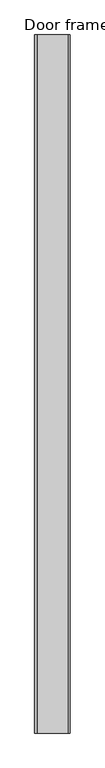
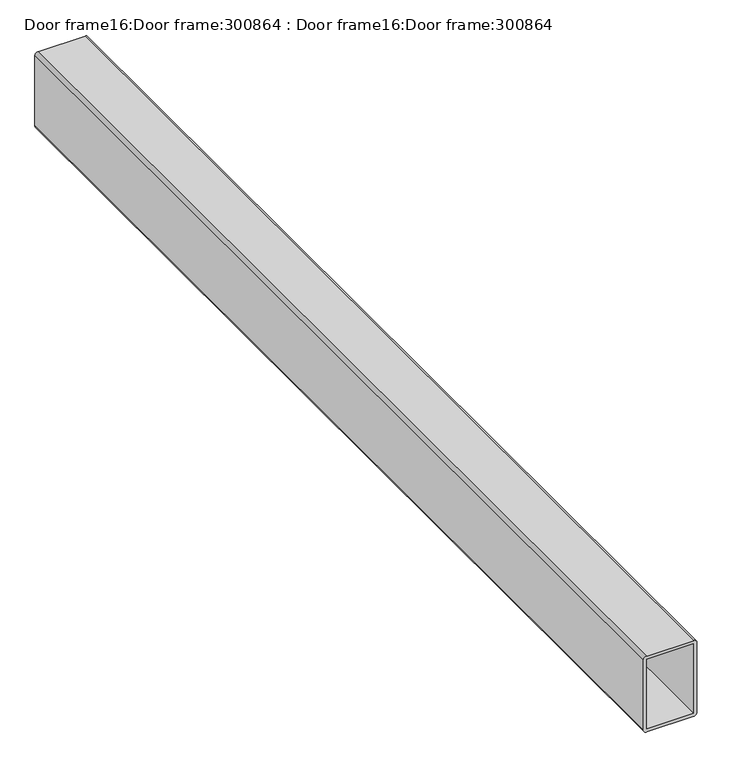
"""IFC4 building model written with IfcOpenShell, lengths in millimetres: proxy geometry, Door frame16:Door frame:300864 : Door frame16:Door frame:300864."""

from ifc_helpers import new_model, si_unit, point, frame, frame_2d, origin, place, context, project, spatial, polyline, circle_curve, trimmed, segment, composite_curve, outline, extrude, source, transform, mapped, element, save


def door_frame16_door_frame_300864_door_frame16_door_frame_4405bbaf(model_context):
    return source(origin(), model_context, "Body", "SweptSolid", [
        extrude(outline(composite_curve([segment(trimmed(circle_curve(frame_2d((34862.2275473, -3620.837526)), 6.35), [point((34862.2275473, -3627.187526))], [point((34855.8775473, -3620.837526))], False, "CARTESIAN"), True, "CONTINUOUS"), segment(polyline([(34855.8775473, -3620.837526), (34855.8775473, -3531.937526)]), True, "CONTINUOUS"), segment(trimmed(circle_curve(frame_2d((34862.2275473, -3531.937526)), 6.35), [point((34855.8775473, -3531.937526))], [point((34862.2275473, -3525.587526))], False, "CARTESIAN"), True, "CONTINUOUS"), segment(polyline([(34862.2275473, -3525.587526), (35001.9275473, -3525.587526)]), True, "CONTINUOUS"), segment(trimmed(circle_curve(frame_2d((35001.9275473, -3531.937526)), 6.35), [point((35001.9275473, -3525.587526))], [point((35008.2775473, -3531.937526))], False, "CARTESIAN"), True, "CONTINUOUS"), segment(polyline([(35008.2775473, -3531.937526), (35008.2775473, -3620.837526)]), True, "CONTINUOUS"), segment(trimmed(circle_curve(frame_2d((35001.9275473, -3620.837526)), 6.35), [point((35008.2775473, -3620.837526))], [point((35001.9275473, -3627.187526))], False, "CARTESIAN"), True, "CONTINUOUS"), segment(polyline([(35001.9275473, -3627.187526), (34862.2275473, -3627.187526)]), True, "CONTINUOUS")], self_intersect=False), holes=[polyline([(35001.7775473, -3620.687526), (35001.7775473, -3532.087526), (34862.3775473, -3532.087526), (34862.3775473, -3620.687526), (35001.7775473, -3620.687526)])]), frame((0.0, 4838.7838655, 0.0), z_axis=(0.0, 1.0, 0.0), x_axis=(0.0, 0.0, 1.0)), (0.0, 0.0, 1.0), 2000.0),
    ])


if __name__ == "__main__":
    model = new_model("IFC4")
    model_context = context("Model", 3, world=origin())
    ifc_project = project(units=[si_unit("LENGTHUNIT", "METRE", prefix="MILLI")], contexts=[model_context])
    site = spatial("IfcSite", under=ifc_project)
    building = spatial("IfcBuilding", under=site)
    placement = place(None, origin())
    door_frame16_door_frame_300864_door_frame16_door_frame_shape = door_frame16_door_frame_300864_door_frame16_door_frame_4405bbaf(model_context)
    element("IfcBuildingElementProxy", 1, Name="Door frame16:Door frame:300864 : Door frame16:Door frame:300864", ObjectType="Door frame16:Door frame:300864 : Door frame16:Door frame:300864", at=placement, inside=building, context=model_context, shape_type="MappedRepresentation", body=[
        mapped(door_frame16_door_frame_300864_door_frame16_door_frame_shape, transform((0.0, 0.0, 0.0), x_axis=(1.0, 0.0, 0.0), y_axis=(0.0, 1.0, 0.0), z_axis=(0.0, 0.0, 1.0))),
    ])
    save(model, "model.ifc")

# Revit data of these elements
# Type "Door frame16:Door frame:300864 : Door frame16:Door frame:300864"
#   NameOverride = "Door frame16:Door frame:300864"
#   ObjectTypeOverride = "Door frame16:Door frame"
#   Reference = "Door frame"
#   Category = "Generic Models"
#   Tag = "300864"
# Element 1 (IfcBuildingElementProxy, "Door frame16:Door frame:300864 : Door frame16:Door frame:300864")
#   Materials on its faces: "TUBE STEEL PROFILE - METALIZED, PRIMED & PAINTED (COLOR PER ARCHITECT)"
# Materials
#   "TUBE STEEL PROFILE - METALIZED, PRIMED & PAINTED (COLOR PER ARCHITECT)": class "Unassigned", colour RGB 128 128 128, transparency 0
